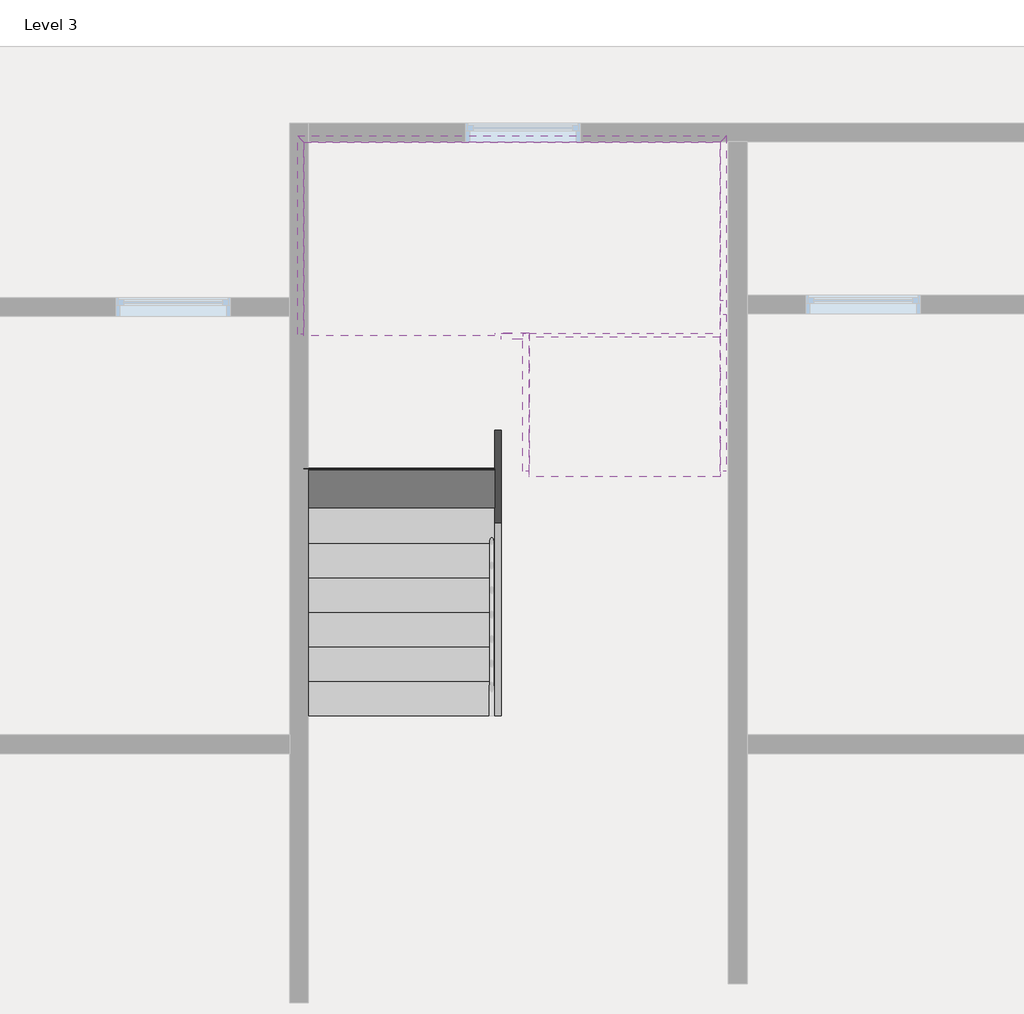
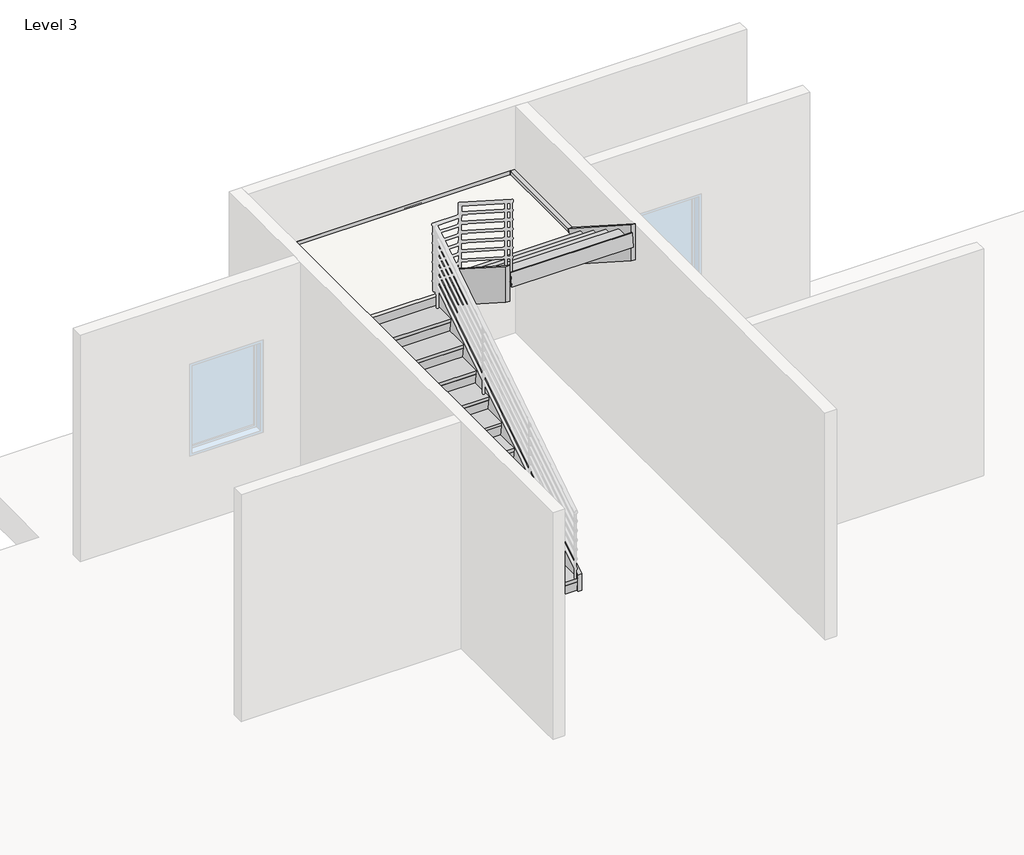
# One storey, part 7 of 7: 8 members, 2 stair flights, 1 slab.
"""IFC4 building model written with IfcOpenShell, lengths in millimetres."""

import ifcopenshell
import ifcopenshell.guid

model = None  # the IFC model being written
_history = None  # IfcOwnerHistory: only IFC2X3 demands one
_inside = {}  # id of a spatial element -> (the spatial element, [elements in it])
_under = {}  # id of a project, library or spatial element -> (it, [spatial elements below it])
_declared = {}  # id of a project -> (the project, [libraries it declares])
_typed = {}  # id of a type object -> (the type object, [elements of that type])
_made_of = {}  # id of a material, layer set ... -> (it, [elements and type objects made of it])


def new_model(schema):
    """Start an empty IFC model of exactly this schema.

    Asked for "IFC4X3", IfcOpenShell would pick the latest addendum, in which some entities
    have other attributes; the version numbers below select the first issue.
    IFC2X3 requires an IfcOwnerHistory on every rooted entity: one is made here for all.
    """
    global model, _history
    if schema == "IFC4X3":
        model = ifcopenshell.file(schema_version=(4, 3, 0, 0))
    else:
        model = ifcopenshell.file(schema=schema)
    _inside.clear()
    _under.clear()
    _declared.clear()
    _typed.clear()
    _made_of.clear()
    _history = None
    if model.schema == "IFC2X3":
        org = make("IfcOrganization", Name="unknown")
        user = make(
            "IfcPersonAndOrganization",
            ThePerson=make("IfcPerson", FamilyName="unknown"),
            TheOrganization=org,
        )
        app = make(
            "IfcApplication",
            ApplicationDeveloper=org,
            Version="unknown",
            ApplicationFullName="unknown",
            ApplicationIdentifier="unknown",
        )
        _history = make(
            "IfcOwnerHistory",
            OwningUser=user,
            OwningApplication=app,
            ChangeAction="ADDED",
            CreationDate=0,
        )
    return model


def make(cls, **values):
    """One entity of the class cls with the attributes given. An attribute that is None is left unset."""
    return model.create_entity(
        cls, **{name: value for name, value in values.items() if value is not None}
    )


def rooted(cls, **values):
    """An entity with a GlobalId (a new one), such as an element, a storey or a relation."""
    return make(cls, GlobalId=ifcopenshell.guid.new(), OwnerHistory=_history, **values)


def si_unit(unit_type, name, prefix=None):
    """IfcSIUnit, for example si_unit("LENGTHUNIT", "METRE", prefix="MILLI")."""
    return make("IfcSIUnit", UnitType=unit_type, Prefix=prefix, Name=name)


def assignment(units):
    """IfcUnitAssignment: the units of a project."""
    return None if units is None else make("IfcUnitAssignment", Units=units)


def point(xyz):
    """IfcCartesianPoint."""
    return None if xyz is None else make("IfcCartesianPoint", Coordinates=xyz)


def direction(xyz):
    """IfcDirection."""
    return None if xyz is None else make("IfcDirection", DirectionRatios=xyz)


def frame(location, z_axis=None, x_axis=None):
    """IfcAxis2Placement3D, a coordinate frame: its origin and axes. An axis left out is left unset."""
    return make(
        "IfcAxis2Placement3D",
        Location=point(location),
        Axis=direction(z_axis),
        RefDirection=direction(x_axis),
    )


def origin():
    """The frame at (0, 0, 0) with its axes left unset."""
    return frame((0.0, 0.0, 0.0))


def place(relative_to, where):
    """IfcLocalPlacement: puts the frame where relative to a parent placement (None: the world)."""
    return make(
        "IfcLocalPlacement", PlacementRelTo=relative_to, RelativePlacement=where
    )


def context(
    kind, dimensions, precision=None, world=None, true_north=None, identifier=None
):
    """IfcGeometricRepresentationContext, for example the 3D "Model" context."""
    return make(
        "IfcGeometricRepresentationContext",
        ContextIdentifier=identifier,
        ContextType=kind,
        CoordinateSpaceDimension=dimensions,
        Precision=precision,
        WorldCoordinateSystem=world,
        TrueNorth=true_north,
    )


def project(units=None, contexts=None):
    """IfcProject with its units and contexts."""
    return rooted(
        "IfcProject",
        Name="project",
        RepresentationContexts=contexts,
        UnitsInContext=assignment(units),
    )


def spatial(cls, under=None, at=None, **own):
    """A site, building, storey or space (cls), placed at a placement, below another one or the project."""
    s = rooted(cls, ObjectPlacement=at, **own)
    if under is not None:
        _under.setdefault(under.id(), (under, []))[1].append(s)
    return s


def polyline(points):
    """IfcPolyline through the points."""
    return make("IfcPolyline", Points=[point(p) for p in points])


def outline(outer, holes=None, kind="AREA"):
    """IfcArbitraryClosedProfileDef: a profile drawn as a closed curve; with holes, ...WithVoids."""
    if holes is None:
        return make("IfcArbitraryClosedProfileDef", ProfileType=kind, OuterCurve=outer)
    return make(
        "IfcArbitraryProfileDefWithVoids",
        ProfileType=kind,
        OuterCurve=outer,
        InnerCurves=holes,
    )


def extrude(swept, where, along, depth):
    """IfcExtrudedAreaSolid: the profile swept, set in the frame where, extruded along a direction by depth."""
    return make(
        "IfcExtrudedAreaSolid",
        SweptArea=swept,
        Position=where,
        ExtrudedDirection=direction(along),
        Depth=depth,
    )


def faces_of(points, faces, orient=None, outer=None):
    """IfcFace entities. A face is a list of loops; a loop is a list of indices into points, from 0.

    orient and outer hold one flag for each loop. By default every Orientation is true, the
    first loop of a face is its IfcFaceOuterBound and the others are IfcFaceBound.
    """
    made = []
    for i, loops in enumerate(faces):
        bounds = []
        for j, loop in enumerate(loops):
            is_outer = j == 0 if outer is None else outer[i][j]
            bounds.append(
                make(
                    "IfcFaceOuterBound" if is_outer else "IfcFaceBound",
                    Bound=make("IfcPolyLoop", Polygon=[points[k] for k in loop]),
                    Orientation=True if orient is None else orient[i][j],
                )
            )
        made.append(make("IfcFace", Bounds=bounds))
    return made


def faceted_brep(points, faces, orient=None, outer=None, voids=None):
    """IfcFacetedBrep: a solid bounded by flat faces; with voids (closed shells), ...WithVoids."""
    shared = [point(p) for p in points]
    hull = make("IfcClosedShell", CfsFaces=faces_of(shared, faces, orient, outer))
    if voids is None:
        return make("IfcFacetedBrep", Outer=hull)
    return make(
        "IfcFacetedBrepWithVoids",
        Outer=hull,
        Voids=[
            make(cls, CfsFaces=faces_of(shared, fs, o, b)) for cls, fs, o, b in voids
        ],
    )


def shape(context_of_items, identifier, shape_type, items):
    """IfcShapeRepresentation: the items that make up one representation, for example the "Body"."""
    return make(
        "IfcShapeRepresentation",
        ContextOfItems=context_of_items,
        RepresentationIdentifier=identifier,
        RepresentationType=shape_type,
        Items=items,
    )


def source(mapping_origin, context_of_items, identifier, shape_type, items):
    """IfcRepresentationMap: a shape defined once, which mapped items show again and again."""
    return make(
        "IfcRepresentationMap",
        MappingOrigin=mapping_origin,
        MappedRepresentation=shape(context_of_items, identifier, shape_type, items),
    )


def transform(
    local_origin,
    x_axis=None,
    y_axis=None,
    z_axis=None,
    scale=None,
    scale2=None,
    scale3=None,
    uniform=True,
):
    """IfcCartesianTransformationOperator3D, or its non-uniform kind. x_axis, y_axis, z_axis: its Axis1, 2, 3."""
    if uniform:
        return make(
            "IfcCartesianTransformationOperator3D",
            Axis1=direction(x_axis),
            Axis2=direction(y_axis),
            LocalOrigin=point(local_origin),
            Scale=scale,
            Axis3=direction(z_axis),
        )
    return make(
        "IfcCartesianTransformationOperator3DnonUniform",
        Axis1=direction(x_axis),
        Axis2=direction(y_axis),
        LocalOrigin=point(local_origin),
        Scale=scale,
        Axis3=direction(z_axis),
        Scale2=scale2,
        Scale3=scale3,
    )


def mapped(mapping_source, mapping_target):
    """IfcMappedItem: shows the shape of a source again, moved by a transform."""
    return make(
        "IfcMappedItem", MappingSource=mapping_source, MappingTarget=mapping_target
    )


def made_of(thing, what):
    """Note that an element or type object is made of a material, layer set ...; save() writes the relation."""
    if what is not None:
        _made_of.setdefault(what.id(), (what, []))[1].append(thing)
    return thing


def element(
    cls,
    number,
    at=None,
    inside=None,
    cuts=None,
    type_object=None,
    material=None,
    context=None,
    identifier="Body",
    shape_type=None,
    held_by="IfcProductDefinitionShape",
    body=None,
    shapes=None,
    **own,
):
    """One element of the class cls, such as IfcWall. Its Tag is "e" and its number.

    at: its placement. inside: the storey or other place that contains it. cuts: it is an
    opening in that element (IfcRelVoidsElement). A single representation is given by context,
    identifier, shape_type and body (its items); several are given by shapes. held_by: the class
    of the entity that holds the representations. save() writes the other relations.
    """
    e = rooted(cls, Tag="e%d" % number, ObjectPlacement=at, **own)
    if body is not None:
        shapes = [shape(context, identifier, shape_type, body)]
    if shapes is not None:
        e.Representation = make(held_by, Representations=shapes)
    if inside is not None:
        _inside.setdefault(inside.id(), (inside, []))[1].append(e)
    if cuts is not None:
        rooted(
            "IfcRelVoidsElement", RelatingBuildingElement=cuts, RelatedOpeningElement=e
        )
    if type_object is not None:
        _typed.setdefault(type_object.id(), (type_object, []))[1].append(e)
    return made_of(e, material)


def aggregate(whole, parts):
    """IfcRelAggregates: a whole, such as a stair, and the parts it consists of."""
    return rooted("IfcRelAggregates", RelatingObject=whole, RelatedObjects=parts)


def save(model, path):
    """Write the relations noted so far, then the file.

    IfcRelAggregates (storeys below a building ...), IfcRelContainedInSpatialStructure (elements
    in a storey), IfcRelDefinesByType, IfcRelAssociatesMaterial and IfcRelDeclares: one each for
    every whole, place, type object, material and project.
    """
    for whole, parts in _under.values():
        aggregate(whole, parts)
    for where, things in _inside.values():
        rooted(
            "IfcRelContainedInSpatialStructure",
            RelatedElements=things,
            RelatingStructure=where,
        )
    for kind, things in _typed.values():
        rooted("IfcRelDefinesByType", RelatedObjects=things, RelatingType=kind)
    for what, things in _made_of.values():
        rooted("IfcRelAssociatesMaterial", RelatedObjects=things, RelatingMaterial=what)
    for by, libraries in _declared.values():
        rooted("IfcRelDeclares", RelatingContext=by, RelatedDefinitions=libraries)
    model.write(path)


def non_monolithic_landing_f178d996(model_context):
    return source(origin(), model_context, "Body", "Brep", [
        faceted_brep([(-226.7120949, 7307.4781803, 8617.6470588), (-226.7120949, 7300.3948469, 8567.6470588), (1293.2879051, 7300.3948469, 8567.6470588), (1293.2879051, 7307.4781803, 8617.6470588), (-499.4393676, 7309.7509075, 8617.6470588), (-499.4393676, 7332.4781803, 8617.6470588), (-226.7120949, 7332.4781803, 8617.6470588), (1293.2879051, 7332.4781803, 8617.6470588), (1293.2879051, 8852.4781803, 8617.6470588), (-2019.4393676, 8852.4781803, 8617.6470588), (-2019.4393676, 7309.7509075, 8617.6470588), (-226.7120949, 7332.4781803, 8567.6470588), (-499.4393676, 7332.4781803, 8567.6470588), (-499.4393676, 7316.8342409, 8567.6470588), (-2019.4393676, 7316.8342409, 8567.6470588), (-2019.4393676, 8852.4781803, 8567.6470588), (1293.2879051, 8852.4781803, 8567.6470588), (1293.2879051, 7332.4781803, 8567.6470588)], [[[0, 1, 2, 3]], [[4, 5, 6, 0, 3, 7, 8, 9, 10]], [[11, 12, 13, 14, 15, 16, 17, 2, 1]], [[5, 4, 13, 12]], [[6, 5, 12, 11]], [[0, 6, 11, 1]], [[7, 3, 2, 17]], [[8, 7, 17, 16]], [[9, 8, 16, 15]], [[10, 9, 15, 14]], [[4, 10, 14, 13]]]),
    ])


def stair_flight_50mm_tread_25mm_nosing_13mm_riser_b2627bcb(model_context):
    return source(origin(), model_context, "Body", "Brep", [
        faceted_brep([(-499.4393676, 4584.7509075, 6676.4705882), (-499.4393676, 4591.8342409, 6626.4705882), (-2019.4393676, 4591.8342409, 6626.4705882), (-2019.4393676, 4584.7509075, 6676.4705882), (-2019.4393676, 4284.7509075, 6676.4705882), (-499.4393676, 4284.7509075, 6676.4705882), (-499.4393676, 4291.8342409, 6626.4705882), (-2019.4393676, 4291.8342409, 6626.4705882)], [[[0, 1, 2, 3]], [[3, 4, 5, 0]], [[2, 1, 6, 7]], [[4, 3, 2, 7]], [[0, 5, 6, 1]], [[5, 4, 7, 6]]]),
        faceted_brep([(-499.4393676, 4291.8342409, 6626.4705882), (-499.4393676, 4309.7509075, 6500.0), (-499.4393676, 4322.3757185, 6500.0), (-499.4393676, 4304.4590518, 6626.4705882), (-2019.4393676, 4291.8342409, 6626.4705882), (-2019.4393676, 4304.4590518, 6626.4705882), (-2019.4393676, 4322.3757185, 6500.0), (-2019.4393676, 4309.7509075, 6500.0)], [[[0, 1, 2, 3]], [[4, 5, 6, 7]], [[1, 0, 4, 7]], [[2, 1, 7, 6]], [[3, 2, 6, 5]], [[0, 3, 5, 4]]]),
        faceted_brep([(-499.4393676, 4566.8342409, 6802.9411765), (-499.4393676, 4591.8342409, 6626.4705882), (-499.4393676, 4604.4590518, 6626.4705882), (-499.4393676, 4579.4590518, 6802.9411765), (-2019.4393676, 4566.8342409, 6802.9411765), (-2019.4393676, 4579.4590518, 6802.9411765), (-2019.4393676, 4604.4590518, 6626.4705882), (-2019.4393676, 4591.8342409, 6626.4705882)], [[[0, 1, 2, 3]], [[4, 5, 6, 7]], [[1, 0, 4, 7]], [[2, 1, 7, 6]], [[3, 2, 6, 5]], [[0, 3, 5, 4]]]),
        faceted_brep([(-2019.4393676, 4859.7509075, 6852.9411765), (-2019.4393676, 4559.7509075, 6852.9411765), (-499.4393676, 4559.7509075, 6852.9411765), (-499.4393676, 4859.7509075, 6852.9411765), (-2019.4393676, 4866.8342409, 6802.9411765), (-499.4393676, 4866.8342409, 6802.9411765), (-499.4393676, 4566.8342409, 6802.9411765), (-2019.4393676, 4566.8342409, 6802.9411765)], [[[0, 1, 2, 3]], [[4, 5, 6, 7]], [[1, 0, 4, 7]], [[3, 2, 6, 5]], [[3, 5, 4, 0]], [[2, 1, 7, 6]]]),
        faceted_brep([(-499.4393676, 4841.8342409, 6979.4117647), (-499.4393676, 4866.8342409, 6802.9411765), (-499.4393676, 4879.4590518, 6802.9411765), (-499.4393676, 4854.4590518, 6979.4117647), (-2019.4393676, 4841.8342409, 6979.4117647), (-2019.4393676, 4854.4590518, 6979.4117647), (-2019.4393676, 4879.4590518, 6802.9411765), (-2019.4393676, 4866.8342409, 6802.9411765)], [[[0, 1, 2, 3]], [[4, 5, 6, 7]], [[1, 0, 4, 7]], [[2, 1, 7, 6]], [[3, 2, 6, 5]], [[0, 3, 5, 4]]]),
        faceted_brep([(-2019.4393676, 5134.7509075, 7029.4117647), (-2019.4393676, 4834.7509075, 7029.4117647), (-499.4393676, 4834.7509075, 7029.4117647), (-499.4393676, 5134.7509075, 7029.4117647), (-2019.4393676, 5141.8342409, 6979.4117647), (-499.4393676, 5141.8342409, 6979.4117647), (-499.4393676, 4841.8342409, 6979.4117647), (-2019.4393676, 4841.8342409, 6979.4117647)], [[[0, 1, 2, 3]], [[4, 5, 6, 7]], [[1, 0, 4, 7]], [[3, 2, 6, 5]], [[3, 5, 4, 0]], [[2, 1, 7, 6]]]),
        faceted_brep([(-499.4393676, 5116.8342409, 7155.8823529), (-499.4393676, 5141.8342409, 6979.4117647), (-499.4393676, 5154.4590518, 6979.4117647), (-499.4393676, 5129.4590518, 7155.8823529), (-2019.4393676, 5116.8342409, 7155.8823529), (-2019.4393676, 5129.4590518, 7155.8823529), (-2019.4393676, 5154.4590518, 6979.4117647), (-2019.4393676, 5141.8342409, 6979.4117647)], [[[0, 1, 2, 3]], [[4, 5, 6, 7]], [[1, 0, 4, 7]], [[2, 1, 7, 6]], [[3, 2, 6, 5]], [[0, 3, 5, 4]]]),
        faceted_brep([(-2019.4393676, 5409.7509075, 7205.8823529), (-2019.4393676, 5109.7509075, 7205.8823529), (-499.4393676, 5109.7509075, 7205.8823529), (-499.4393676, 5409.7509075, 7205.8823529), (-2019.4393676, 5416.8342409, 7155.8823529), (-499.4393676, 5416.8342409, 7155.8823529), (-499.4393676, 5116.8342409, 7155.8823529), (-2019.4393676, 5116.8342409, 7155.8823529)], [[[0, 1, 2, 3]], [[4, 5, 6, 7]], [[1, 0, 4, 7]], [[3, 2, 6, 5]], [[3, 5, 4, 0]], [[2, 1, 7, 6]]]),
        faceted_brep([(-499.4393676, 5391.8342409, 7332.3529412), (-499.4393676, 5416.8342409, 7155.8823529), (-499.4393676, 5429.4590518, 7155.8823529), (-499.4393676, 5404.4590518, 7332.3529412), (-2019.4393676, 5391.8342409, 7332.3529412), (-2019.4393676, 5404.4590518, 7332.3529412), (-2019.4393676, 5429.4590518, 7155.8823529), (-2019.4393676, 5416.8342409, 7155.8823529)], [[[0, 1, 2, 3]], [[4, 5, 6, 7]], [[1, 0, 4, 7]], [[2, 1, 7, 6]], [[3, 2, 6, 5]], [[0, 3, 5, 4]]]),
        faceted_brep([(-2019.4393676, 5684.7509075, 7382.3529412), (-2019.4393676, 5384.7509075, 7382.3529412), (-499.4393676, 5384.7509075, 7382.3529412), (-499.4393676, 5684.7509075, 7382.3529412), (-2019.4393676, 5691.8342409, 7332.3529412), (-499.4393676, 5691.8342409, 7332.3529412), (-499.4393676, 5391.8342409, 7332.3529412), (-2019.4393676, 5391.8342409, 7332.3529412)], [[[0, 1, 2, 3]], [[4, 5, 6, 7]], [[1, 0, 4, 7]], [[3, 2, 6, 5]], [[3, 5, 4, 0]], [[2, 1, 7, 6]]]),
        faceted_brep([(-499.4393676, 5666.8342409, 7508.8235294), (-499.4393676, 5691.8342409, 7332.3529412), (-499.4393676, 5704.4590518, 7332.3529412), (-499.4393676, 5679.4590518, 7508.8235294), (-2019.4393676, 5666.8342409, 7508.8235294), (-2019.4393676, 5679.4590518, 7508.8235294), (-2019.4393676, 5704.4590518, 7332.3529412), (-2019.4393676, 5691.8342409, 7332.3529412)], [[[0, 1, 2, 3]], [[4, 5, 6, 7]], [[1, 0, 4, 7]], [[2, 1, 7, 6]], [[3, 2, 6, 5]], [[0, 3, 5, 4]]]),
        faceted_brep([(-2019.4393676, 5959.7509075, 7558.8235294), (-2019.4393676, 5659.7509075, 7558.8235294), (-499.4393676, 5659.7509075, 7558.8235294), (-499.4393676, 5959.7509075, 7558.8235294), (-2019.4393676, 5966.8342409, 7508.8235294), (-499.4393676, 5966.8342409, 7508.8235294), (-499.4393676, 5666.8342409, 7508.8235294), (-2019.4393676, 5666.8342409, 7508.8235294)], [[[0, 1, 2, 3]], [[4, 5, 6, 7]], [[1, 0, 4, 7]], [[3, 2, 6, 5]], [[3, 5, 4, 0]], [[2, 1, 7, 6]]]),
        faceted_brep([(-499.4393676, 5941.8342409, 7685.2941176), (-499.4393676, 5966.8342409, 7508.8235294), (-499.4393676, 5979.4590518, 7508.8235294), (-499.4393676, 5954.4590518, 7685.2941176), (-2019.4393676, 5941.8342409, 7685.2941176), (-2019.4393676, 5954.4590518, 7685.2941176), (-2019.4393676, 5979.4590518, 7508.8235294), (-2019.4393676, 5966.8342409, 7508.8235294)], [[[0, 1, 2, 3]], [[4, 5, 6, 7]], [[1, 0, 4, 7]], [[2, 1, 7, 6]], [[3, 2, 6, 5]], [[0, 3, 5, 4]]]),
        faceted_brep([(-2019.4393676, 6234.7509075, 7735.2941176), (-2019.4393676, 5934.7509075, 7735.2941176), (-499.4393676, 5934.7509075, 7735.2941176), (-499.4393676, 6234.7509075, 7735.2941176), (-2019.4393676, 6241.8342409, 7685.2941176), (-499.4393676, 6241.8342409, 7685.2941176), (-499.4393676, 5941.8342409, 7685.2941176), (-2019.4393676, 5941.8342409, 7685.2941176)], [[[0, 1, 2, 3]], [[4, 5, 6, 7]], [[1, 0, 4, 7]], [[3, 2, 6, 5]], [[3, 5, 4, 0]], [[2, 1, 7, 6]]]),
        faceted_brep([(-499.4393676, 6216.8342409, 7861.7647059), (-499.4393676, 6241.8342409, 7685.2941176), (-499.4393676, 6254.4590518, 7685.2941176), (-499.4393676, 6229.4590518, 7861.7647059), (-2019.4393676, 6216.8342409, 7861.7647059), (-2019.4393676, 6229.4590518, 7861.7647059), (-2019.4393676, 6254.4590518, 7685.2941176), (-2019.4393676, 6241.8342409, 7685.2941176)], [[[0, 1, 2, 3]], [[4, 5, 6, 7]], [[1, 0, 4, 7]], [[2, 1, 7, 6]], [[3, 2, 6, 5]], [[0, 3, 5, 4]]]),
        faceted_brep([(-2019.4393676, 6509.7509075, 7911.7647059), (-2019.4393676, 6209.7509075, 7911.7647059), (-499.4393676, 6209.7509075, 7911.7647059), (-499.4393676, 6509.7509075, 7911.7647059), (-2019.4393676, 6516.8342409, 7861.7647059), (-499.4393676, 6516.8342409, 7861.7647059), (-499.4393676, 6216.8342409, 7861.7647059), (-2019.4393676, 6216.8342409, 7861.7647059)], [[[0, 1, 2, 3]], [[4, 5, 6, 7]], [[1, 0, 4, 7]], [[3, 2, 6, 5]], [[3, 5, 4, 0]], [[2, 1, 7, 6]]]),
        faceted_brep([(-499.4393676, 6491.8342409, 8038.2352941), (-499.4393676, 6516.8342409, 7861.7647059), (-499.4393676, 6529.4590518, 7861.7647059), (-499.4393676, 6504.4590518, 8038.2352941), (-2019.4393676, 6491.8342409, 8038.2352941), (-2019.4393676, 6504.4590518, 8038.2352941), (-2019.4393676, 6529.4590518, 7861.7647059), (-2019.4393676, 6516.8342409, 7861.7647059)], [[[0, 1, 2, 3]], [[4, 5, 6, 7]], [[1, 0, 4, 7]], [[2, 1, 7, 6]], [[3, 2, 6, 5]], [[0, 3, 5, 4]]]),
        faceted_brep([(-2019.4393676, 6784.7509075, 8088.2352941), (-2019.4393676, 6484.7509075, 8088.2352941), (-499.4393676, 6484.7509075, 8088.2352941), (-499.4393676, 6784.7509075, 8088.2352941), (-2019.4393676, 6791.8342409, 8038.2352941), (-499.4393676, 6791.8342409, 8038.2352941), (-499.4393676, 6491.8342409, 8038.2352941), (-2019.4393676, 6491.8342409, 8038.2352941)], [[[0, 1, 2, 3]], [[4, 5, 6, 7]], [[1, 0, 4, 7]], [[3, 2, 6, 5]], [[3, 5, 4, 0]], [[2, 1, 7, 6]]]),
        faceted_brep([(-499.4393676, 6766.8342409, 8214.7058824), (-499.4393676, 6791.8342409, 8038.2352941), (-499.4393676, 6804.4590518, 8038.2352941), (-499.4393676, 6779.4590518, 8214.7058824), (-2019.4393676, 6766.8342409, 8214.7058824), (-2019.4393676, 6779.4590518, 8214.7058824), (-2019.4393676, 6804.4590518, 8038.2352941), (-2019.4393676, 6791.8342409, 8038.2352941)], [[[0, 1, 2, 3]], [[4, 5, 6, 7]], [[1, 0, 4, 7]], [[2, 1, 7, 6]], [[3, 2, 6, 5]], [[0, 3, 5, 4]]]),
        faceted_brep([(-2019.4393676, 7059.7509075, 8264.7058824), (-2019.4393676, 6759.7509075, 8264.7058824), (-499.4393676, 6759.7509075, 8264.7058824), (-499.4393676, 7059.7509075, 8264.7058824), (-2019.4393676, 7066.8342409, 8214.7058824), (-499.4393676, 7066.8342409, 8214.7058824), (-499.4393676, 6766.8342409, 8214.7058824), (-2019.4393676, 6766.8342409, 8214.7058824)], [[[0, 1, 2, 3]], [[4, 5, 6, 7]], [[1, 0, 4, 7]], [[3, 2, 6, 5]], [[3, 5, 4, 0]], [[2, 1, 7, 6]]]),
        faceted_brep([(-499.4393676, 7316.8342409, 8567.6470588), (-499.4393676, 7341.8342409, 8391.1764706), (-499.4393676, 7354.4590518, 8391.1764706), (-499.4393676, 7329.4590518, 8567.6470588), (-2019.4393676, 7316.8342409, 8567.6470588), (-2019.4393676, 7329.4590518, 8567.6470588), (-2019.4393676, 7354.4590518, 8391.1764706), (-2019.4393676, 7341.8342409, 8391.1764706)], [[[0, 1, 2, 3]], [[4, 5, 6, 7]], [[1, 0, 4, 7]], [[2, 1, 7, 6]], [[3, 2, 6, 5]], [[0, 3, 5, 4]]]),
        faceted_brep([(-499.4393676, 7041.8342409, 8391.1764706), (-499.4393676, 7066.8342409, 8214.7058824), (-499.4393676, 7079.4590518, 8214.7058824), (-499.4393676, 7054.4590518, 8391.1764706), (-2019.4393676, 7041.8342409, 8391.1764706), (-2019.4393676, 7054.4590518, 8391.1764706), (-2019.4393676, 7079.4590518, 8214.7058824), (-2019.4393676, 7066.8342409, 8214.7058824)], [[[0, 1, 2, 3]], [[4, 5, 6, 7]], [[1, 0, 4, 7]], [[2, 1, 7, 6]], [[3, 2, 6, 5]], [[0, 3, 5, 4]]]),
        faceted_brep([(-2019.4393676, 7334.7509075, 8441.1764706), (-2019.4393676, 7309.7509075, 8441.1764706), (-2019.4393676, 7034.7509075, 8441.1764706), (-499.4393676, 7034.7509075, 8441.1764706), (-499.4393676, 7334.7509075, 8441.1764706), (-2019.4393676, 7341.8342409, 8391.1764706), (-499.4393676, 7341.8342409, 8391.1764706), (-499.4393676, 7041.8342409, 8391.1764706), (-2019.4393676, 7041.8342409, 8391.1764706), (-2019.4393676, 7309.7509075, 8391.1764706)], [[[0, 1, 2, 3, 4]], [[5, 6, 7, 8, 9]], [[1, 0, 5, 9]], [[2, 1, 9, 8]], [[4, 3, 7, 6]], [[4, 6, 5, 0]], [[3, 2, 8, 7]]]),
    ])


def stair_flight_50mm_tread_25mm_nosing_13mm_riser_53dc4827(model_context):
    return source(origin(), model_context, "Body", "SweptSolid", [
        extrude(outline(polyline([(7032.4781803, 8794.1176471), (7332.4781803, 8794.1176471), (7325.3948469, 8744.1176471), (7025.3948469, 8744.1176471), (7032.4781803, 8794.1176471)])), frame((-226.7120949, 0.0, 0.0), z_axis=(1.0, 0.0, 0.0), x_axis=(0.0, 1.0, 0.0)), (0.0, 0.0, 1.0), 1520.0),
        extrude(outline(polyline([(7325.3948469, 8744.1176471), (7300.3948469, 8567.6470588), (7287.770036, 8567.6470588), (7312.770036, 8744.1176471), (7325.3948469, 8744.1176471)])), frame((-226.7120949, 0.0, 0.0), z_axis=(1.0, 0.0, 0.0), x_axis=(0.0, 1.0, 0.0)), (0.0, 0.0, 1.0), 1520.0),
        extrude(outline(polyline([(7050.3948469, 8920.5882353), (7025.3948469, 8744.1176471), (7012.770036, 8744.1176471), (7037.770036, 8920.5882353), (7050.3948469, 8920.5882353)])), frame((-226.7120949, 0.0, 0.0), z_axis=(1.0, 0.0, 0.0), x_axis=(0.0, 1.0, 0.0)), (0.0, 0.0, 1.0), 1520.0),
        extrude(outline(polyline([(6757.4781803, 8970.5882353), (7057.4781803, 8970.5882353), (7050.3948469, 8920.5882353), (6750.3948469, 8920.5882353), (6757.4781803, 8970.5882353)])), frame((-226.7120949, 0.0, 0.0), z_axis=(1.0, 0.0, 0.0), x_axis=(0.0, 1.0, 0.0)), (0.0, 0.0, 1.0), 1520.0),
        extrude(outline(polyline([(6775.3948469, 9097.0588235), (6750.3948469, 8920.5882353), (6737.770036, 8920.5882353), (6762.770036, 9097.0588235), (6775.3948469, 9097.0588235)])), frame((-226.7120949, 0.0, 0.0), z_axis=(1.0, 0.0, 0.0), x_axis=(0.0, 1.0, 0.0)), (0.0, 0.0, 1.0), 1520.0),
        extrude(outline(polyline([(6482.4781803, 9147.0588235), (6782.4781803, 9147.0588235), (6775.3948469, 9097.0588235), (6475.3948469, 9097.0588235), (6482.4781803, 9147.0588235)])), frame((-226.7120949, 0.0, 0.0), z_axis=(1.0, 0.0, 0.0), x_axis=(0.0, 1.0, 0.0)), (0.0, 0.0, 1.0), 1520.0),
        extrude(outline(polyline([(6500.3948469, 9273.5294118), (6475.3948469, 9097.0588235), (6462.770036, 9097.0588235), (6487.770036, 9273.5294118), (6500.3948469, 9273.5294118)])), frame((-226.7120949, 0.0, 0.0), z_axis=(1.0, 0.0, 0.0), x_axis=(0.0, 1.0, 0.0)), (0.0, 0.0, 1.0), 1520.0),
        extrude(outline(polyline([(6225.3948469, 9450.0), (6200.3948469, 9273.5294118), (6187.770036, 9273.5294118), (6212.770036, 9450.0), (6225.3948469, 9450.0)])), frame((-226.7120949, 0.0, 0.0), z_axis=(1.0, 0.0, 0.0), x_axis=(0.0, 1.0, 0.0)), (0.0, 0.0, 1.0), 1520.0),
        extrude(outline(polyline([(6207.4781803, 9323.5294118), (6507.4781803, 9323.5294118), (6500.3948469, 9273.5294118), (6200.3948469, 9273.5294118), (6207.4781803, 9323.5294118)])), frame((-226.7120949, 0.0, 0.0), z_axis=(1.0, 0.0, 0.0), x_axis=(0.0, 1.0, 0.0)), (0.0, 0.0, 1.0), 1520.0),
    ])


model = new_model("IFC4")

# Units and contexts
model_context = context("Model", 3, world=origin())
ifc_project = project(units=[si_unit("LENGTHUNIT", "METRE", prefix="MILLI")], contexts=[model_context])

# Site, building, storey
site = spatial("IfcSite", under=ifc_project)
building = spatial("IfcBuilding", under=site)
storey = spatial("IfcBuildingStorey", under=building, Name="Level 3", Elevation=6500.0)

# Members
placement = place(None, origin())
element("IfcMember", 1, ObjectType="Stringer - 50mm Width", at=placement, inside=storey, context=model_context, shape_type="SweptSolid", body=[
    extrude(outline(polyline([(4284.7509075, 6500.0), (4284.7509075, 6715.9811749), (7322.0354678, 8665.0407858), (7439.3399977, 8265.0407858), (4688.8181065, 6500.0), (4284.7509075, 6500.0)])), frame((-2069.4393676, 0.0, 0.0), z_axis=(1.0, 0.0, 0.0), x_axis=(0.0, 1.0, 0.0)), (0.0, 0.0, 1.0), 50.0),
])
element("IfcMember", 2, ObjectType="Stringer - 50mm Width", at=placement, inside=storey, context=model_context, shape_type="SweptSolid", body=[
    extrude(outline(polyline([(4284.7509075, 6500.0), (4284.7509075, 6715.9811749), (7322.0354678, 8665.0407858), (7332.4781803, 8665.0407858), (7332.4781803, 8196.4663575), (4688.8181065, 6500.0), (4284.7509075, 6500.0)])), frame((-499.4393676, 0.0, 0.0), z_axis=(1.0, 0.0, 0.0), x_axis=(0.0, 1.0, 0.0)), (0.0, 0.0, 1.0), 50.0),
])
element("IfcMember", 3, ObjectType="Stringer - 50mm Width", at=placement, inside=storey, context=model_context, shape_type="SweptSolid", body=[
    extrude(outline(polyline([(7595.19362, 8665.0407858), (7477.8890902, 8265.0407858), (6232.4781803, 9064.2349525), (6232.4781803, 9539.5105867), (7595.19362, 8665.0407858)])), frame((1293.2879051, 0.0, 0.0), z_axis=(1.0, 0.0, 0.0), x_axis=(0.0, 1.0, 0.0)), (0.0, 0.0, 1.0), 50.0),
])
element("IfcMember", 4, ObjectType="Stringer - 50mm Width", at=placement, inside=storey, context=model_context, shape_type="SweptSolid", body=[
    extrude(outline(polyline([(7332.4781803, 8833.6282338), (7332.4781803, 8358.3525996), (6232.4781803, 9064.2349525), (6232.4781803, 9539.5105867), (7332.4781803, 8833.6282338)])), frame((-276.7120949, 0.0, 0.0), z_axis=(1.0, 0.0, 0.0), x_axis=(0.0, 1.0, 0.0)), (0.0, 0.0, 1.0), 50.0),
])
element("IfcMember", 5, ObjectType="Stringer - 50mm Width", at=placement, inside=storey, context=model_context, shape_type="Brep", body=[
    faceted_brep([(1293.2879051, 7595.19362, 8665.0407858), (1343.2879051, 7595.19362, 8665.0407858), (1343.2879051, 8902.4781803, 8665.0407858), (1293.2879051, 8852.4781803, 8665.0407858), (1293.2879051, 7477.8890902, 8265.0407858), (1293.2879051, 8852.4781803, 8265.0407858), (1343.2879051, 7477.8890902, 8265.0407858), (1343.2879051, 8902.4781803, 8265.0407858)], [[[0, 1, 2, 3]], [[4, 0, 3, 5]], [[6, 4, 5, 7]], [[1, 6, 7, 2]], [[1, 0, 4, 6]], [[2, 7, 5, 3]]]),
])
element("IfcMember", 6, ObjectType="Stringer - 50mm Width", at=placement, inside=storey, context=model_context, shape_type="SweptSolid", body=[
    extrude(outline(polyline([(1343.2879051, 8902.4781803), (1293.2879051, 8852.4781803), (-2019.4393676, 8852.4781803), (-2069.4393676, 8902.4781803), (1343.2879051, 8902.4781803)])), frame((0.0, 0.0, 8265.0407858), z_axis=(0.0, 0.0, 1.0), x_axis=(1.0, 0.0, 0.0)), (0.0, 0.0, 1.0), 400.0),
])
element("IfcMember", 7, ObjectType="Stringer - 50mm Width", at=placement, inside=storey, context=model_context, shape_type="Brep", body=[
    faceted_brep([(-2019.4393676, 8852.4781803, 8665.0407858), (-2069.4393676, 8902.4781803, 8665.0407858), (-2069.4393676, 7322.0354678, 8665.0407858), (-2019.4393676, 7322.0354678, 8665.0407858), (-2019.4393676, 8852.4781803, 8265.0407858), (-2019.4393676, 7439.3399977, 8265.0407858), (-2069.4393676, 8902.4781803, 8265.0407858), (-2069.4393676, 7439.3399977, 8265.0407858)], [[[0, 1, 2, 3]], [[4, 0, 3, 5]], [[6, 4, 5, 7]], [[1, 6, 7, 2]], [[1, 0, 4, 6]], [[2, 7, 5, 3]]]),
])
element("IfcMember", 8, ObjectType="Stringer - 50mm Width", at=placement, inside=storey, context=model_context, shape_type="SweptSolid", body=[
    extrude(outline(polyline([(-449.4393676, 7282.4781803), (-449.4393676, 7332.4781803), (-276.7120949, 7332.4781803), (-276.7120949, 7282.4781803), (-449.4393676, 7282.4781803)])), frame((0.0, 0.0, 8265.0407858), z_axis=(0.0, 0.0, 1.0), x_axis=(1.0, 0.0, 0.0)), (0.0, 0.0, 1.0), 400.0),
])

# Slab
non_monolithic_landing_shape = non_monolithic_landing_f178d996(model_context)
element("IfcSlab", 9, ObjectType="Non-Monolithic Landing", at=placement, inside=storey, context=model_context, shape_type="MappedRepresentation", body=[
    mapped(non_monolithic_landing_shape, transform((0.0, 0.0, 0.0), x_axis=(1.0, 0.0, 0.0), y_axis=(0.0, 1.0, 0.0), z_axis=(0.0, 0.0, 1.0))),
])

# Stair flights
stair_flight_50mm_tread_25mm_nosing_13mm_riser_shape = stair_flight_50mm_tread_25mm_nosing_13mm_riser_b2627bcb(model_context)
element("IfcStairFlight", 10, ObjectType="50mm Tread 25mm Nosing 13mm Riser", at=placement, inside=storey, context=model_context, shape_type="MappedRepresentation", body=[
    mapped(stair_flight_50mm_tread_25mm_nosing_13mm_riser_shape, transform((0.0, 0.0, 0.0), x_axis=(1.0, 0.0, 0.0), y_axis=(0.0, 1.0, 0.0), z_axis=(0.0, 0.0, 1.0))),
])
stair_flight_50mm_tread_25mm_nosing_13mm_riser_2_shape = stair_flight_50mm_tread_25mm_nosing_13mm_riser_53dc4827(model_context)
element("IfcStairFlight", 11, ObjectType="50mm Tread 25mm Nosing 13mm Riser", at=placement, inside=storey, context=model_context, shape_type="MappedRepresentation", body=[
    mapped(stair_flight_50mm_tread_25mm_nosing_13mm_riser_2_shape, transform((0.0, 0.0, 0.0), x_axis=(1.0, 0.0, 0.0), y_axis=(0.0, 1.0, 0.0), z_axis=(0.0, 0.0, 1.0))),
])

save(model, "model.ifc")

# Revit data of these elements
# Elements 1, 2, 3, 4, 5, 6, 7, 8 (IfcMember, "Stringer - 50mm Width")
#   Phase Created = New Construction
# Element 9 (IfcSlab, "Non-Monolithic Landing")
#   Phase Created = New Construction
# Elements 10, 11 (IfcStairFlight, "50mm Tread 25mm Nosing 13mm Riser")
#   Phase Created = New Construction
